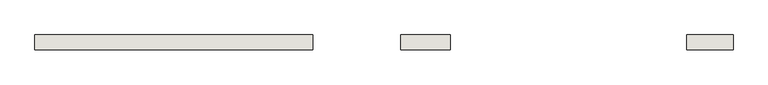
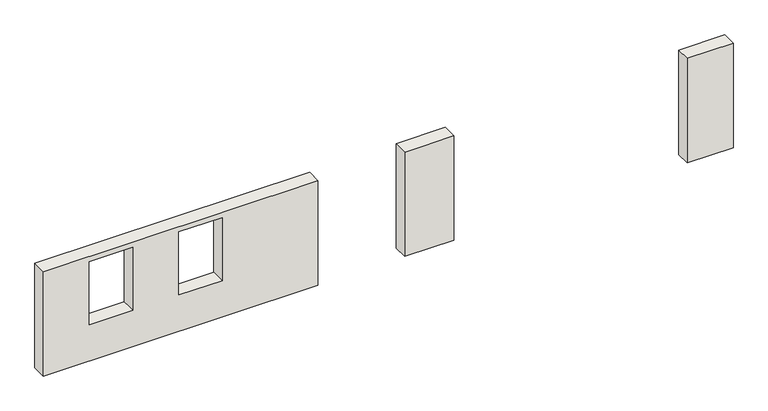
"""IFC4 building model written with IfcOpenShell, lengths in millimetres: wall geometry, 0_3d."""

from ifc_helpers import new_model, si_unit, frame, origin, origin_with_axes, place, context, project, spatial, polyline, outline, extrude, source, transform, mapped, element, save


def wall_c2d978ab(model_context):
    return source(origin(), model_context, "Body", "SweptSolid", [
        extrude(outline(polyline([(16803.259317, 0.0), (16803.259317, 380.0), (18002.8619019, 380.0), (18002.8619019, 0.0), (16803.259317, 0.0)])), origin_with_axes(), (0.0, 0.0, 1.0), 2880.0),
        extrude(outline(polyline([(0.0, 7167.897415), (2880.0, 7167.897415), (2880.0, 0.0), (0.0, 0.0), (0.0, 7167.897415)]), holes=[polyline([(2740.0, 4668.0664986), (1000.0, 4668.0664986), (1000.0, 3533.0664986), (2740.0, 3533.0664986), (2740.0, 4668.0664986)]), polyline([(2740.0, 2334.2006715), (1000.0, 2334.2006715), (1000.0, 1199.2006715), (2740.0, 1199.2006715), (2740.0, 2334.2006715)])]), frame((0.0, 0.0, 0.0), z_axis=(0.0, 1.0, 0.0), x_axis=(0.0, 0.0, 1.0)), (0.0, 0.0, 1.0), 380.0),
        extrude(outline(polyline([(9427.897415, 0.0), (9427.897415, 380.0), (10707.5, 380.0), (10707.5, 0.0), (9427.897415, 0.0)])), origin_with_axes(), (0.0, 0.0, 1.0), 2880.0),
    ])


if __name__ == "__main__":
    model = new_model("IFC4")
    model_context = context("Model", 3, world=origin())
    ifc_project = project(units=[si_unit("LENGTHUNIT", "METRE", prefix="MILLI")], contexts=[model_context])
    site = spatial("IfcSite", under=ifc_project)
    building = spatial("IfcBuilding", under=site)
    placement = place(None, origin())
    wall_shape = wall_c2d978ab(model_context)
    element("IfcWall", 1, ObjectType="0_3d", at=placement, inside=building, context=model_context, shape_type="MappedRepresentation", body=[
        mapped(wall_shape, transform((0.0, 0.0, 0.0), x_axis=(1.0, 0.0, 0.0), y_axis=(0.0, 1.0, 0.0), z_axis=(0.0, 0.0, 1.0))),
    ])
    save(model, "model.ifc")

# Revit data of these elements
# Element 1 (IfcWall, "0_3d")
#   Materials on its faces: "holzschalung"
# Materials
#   "holzschalung": class "Unassigned", colour RGB 128 128 128, transparency 0
